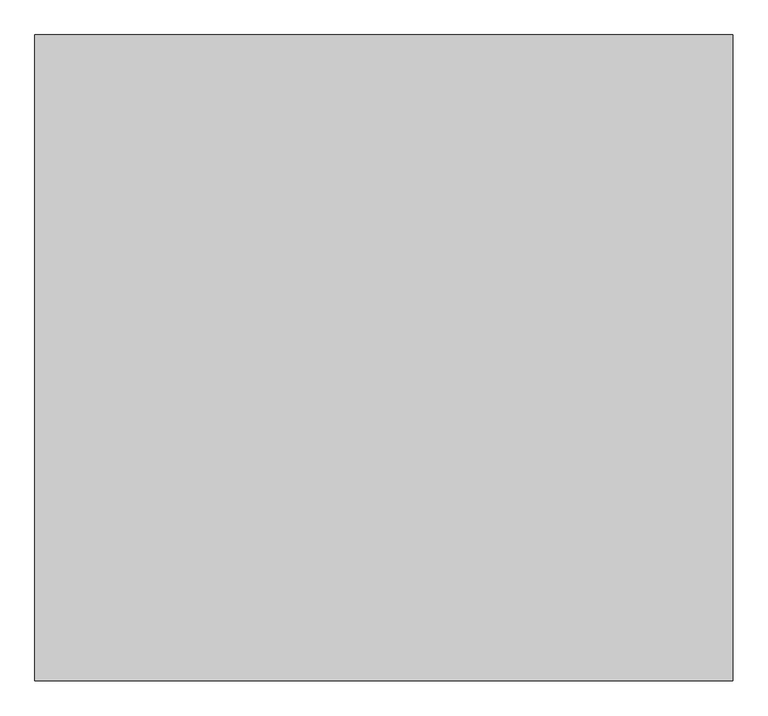
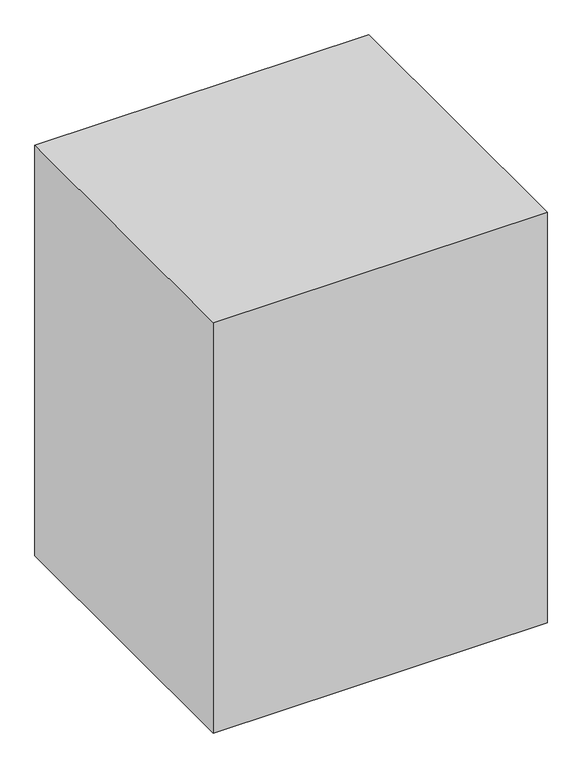
"""IFC4 building model written with IfcOpenShell, lengths in millimetres: proxy geometry, Space Planning Box_hec : Space Planning Box_hec."""

from ifc_helpers import new_model, si_unit, origin, origin_with_axes, place, context, project, spatial, polyline, outline, extrude, source, transform, mapped, element, save


def generic_models_0e92175d(model_context):
    return source(origin(), model_context, "Body", "SweptSolid", [
        extrude(outline(polyline([(2000.0, 1850.0), (2000.0, -1850.0), (-2000.0, -1850.0), (-2000.0, 1850.0), (2000.0, 1850.0)])), origin_with_axes(), (0.0, 0.0, 1.0), 5200.0),
    ])


if __name__ == "__main__":
    model = new_model("IFC4")
    model_context = context("Model", 3, world=origin())
    ifc_project = project(units=[si_unit("LENGTHUNIT", "METRE", prefix="MILLI")], contexts=[model_context])
    site = spatial("IfcSite", under=ifc_project)
    building = spatial("IfcBuilding", under=site)
    placement = place(None, origin())
    generic_models_shape = generic_models_0e92175d(model_context)
    element("IfcBuildingElementProxy", 1, Name="Space Planning Box_hec : Space Planning Box_hec", ObjectType="Space Planning Box_hec : Space Planning Box_hec", at=placement, inside=building, context=model_context, shape_type="MappedRepresentation", body=[
        mapped(generic_models_shape, transform((0.0, 0.0, 0.0), x_axis=(1.0, 0.0, 0.0), y_axis=(0.0, 1.0, 0.0), z_axis=(0.0, 0.0, 1.0))),
    ])
    save(model, "model.ifc")

# Revit data of these elements
# Type "Space Planning Box_hec : Space Planning Box_hec"
#   Type Comments = "..."
#   Room Name [instance default] = "?"
#   Interior Finish [instance default] = ""
#   Exterior Finish [instance default] = ""
#   Department [instance default] = ""
#   Assembly Code = "..."
#   ceiling height [instance default] = 0
#   Width [instance default] = 1524 mm
#   Program Area [instance default] = 0.00 m²
#   Length [instance default] = 1524 mm
#   Height [instance default] = 1524 mm
#   Area [instance default] = 2.32258 m²
#   Fill Color [instance default] = Cyan
#   Default Elevation = 0
# Element 1 (IfcBuildingElementProxy, "Space Planning Box_hec : Space Planning Box_hec")
#   Room Name = "Pantry"
#   Interior Finish = "IW1..N/A,,WB2..N/A,,FL6..N/A,,CL4..N/A"
#   Exterior Finish = "RF1..N/A,,EW1..N/A"
#   Department = "AR"
#   ceiling height = 2700
#   Width = 4000 mm
#   Program Area = 14.80 m²
#   Length = 3700 mm
#   Height = 5200 mm
#   Area = 14.80 m²
#   Materials on its faces: "Cyan"
# Materials
#   "Cyan": class "Generic", colour RGB 0 255 255, transparency 0.2, Cost = 0
